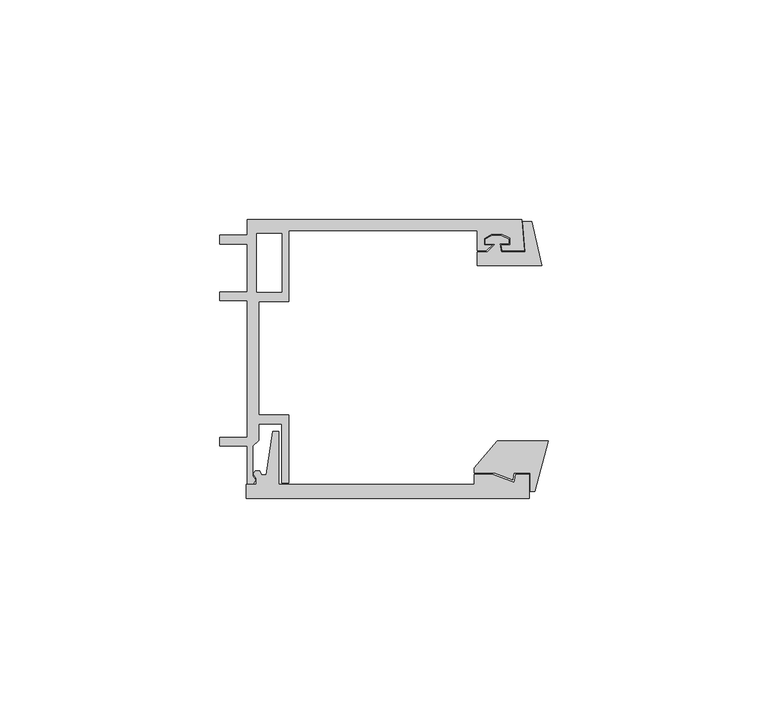
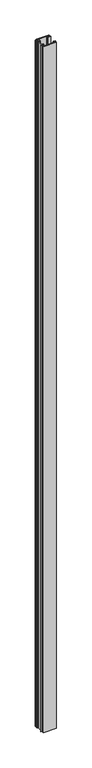
"""IFC4 building model written with IfcOpenShell, lengths in millimetres: proxy geometry, Generic Models 2:Generic Models 2:310765:Generic Models 2:310765 : Generic Models 2:Generic Models 2:310765:69 : Generic Models 2:Generic Models 2:310765:Generic Models 2:310765 : Generic Models 2:Generic Models 2:310765:300385."""

from ifc_helpers import new_model, si_unit, frame, origin, place, context, project, spatial, polyline, outline, extrude, source, transform, mapped, element, save


def generic_models_3473c4d2(model_context):
    return source(origin(), model_context, "Body", "SweptSolid", [
        extrude(outline(polyline([(596192.2839587, -579078.5739799), (596192.7605868, -579079.4334593), (596193.8113738, -579079.4334593), (596195.2258729, -579069.5319653), (596196.5980218, -579069.5319653), (596196.5980218, -579081.6864938), (596241.1250993, -579081.6864938), (596241.1250993, -579079.3741689), (596245.3940068, -579079.3741689), (596250.2558182, -579081.1528804), (596250.5522702, -579079.3741689), (596253.6946604, -579079.3741689), (596253.6946604, -579084.8288841), (596189.1867239, -579084.8288841), (596189.1867239, -579081.6864938), (596191.4990489, -579081.6864938), (596191.4990489, -579080.2786171), (596190.8403865, -579079.2652904), (596191.3340898, -579078.5247354), (596192.2839587, -579078.5739799)])), frame((0.0, 0.0, 1989.1494403), z_axis=(0.0, 0.0, 1.0), x_axis=(1.0, 0.0, 0.0)), (0.0, 0.0, 1.0), 3670.2203961),
        extrude(outline(polyline([(596254.9309933, -579083.2164454), (596253.8923802, -579083.2164454), (596253.8923802, -579079.0835833), (596250.1261424, -579079.0835833), (596249.8691362, -579080.6256201), (596245.6542355, -579079.0835833), (596241.1250993, -579079.0835833), (596241.1250993, -579077.8782793), (596246.3737657, -579071.7849999), (596257.9793788, -579071.7849999), (596254.9309933, -579083.2164454)])), frame((0.0, 0.0, 1989.1494403), z_axis=(0.0, 0.0, 1.0), x_axis=(1.0, 0.0, 0.0)), (0.0, 0.0, 1.0), 3670.2203961),
        extrude(outline(polyline([(596241.8365839, -579023.8783705), (596198.9103467, -579023.8783705), (596198.9103467, -579039.9460643), (596192.0326623, -579039.9460643), (596192.0326623, -579065.8559616), (596198.9103467, -579065.8559616), (596198.9103467, -579081.3307515), (596197.3687968, -579081.3307515), (596197.3687968, -579067.8718346), (596192.0326623, -579067.8718346), (596192.0326623, -579071.6071287), (596190.7282739, -579072.9115171), (596190.7282739, -579079.7299112), (596191.3804681, -579080.6785573), (596190.8468547, -579081.5086227), (596189.4831758, -579081.5086227), (596189.4831758, -579072.9115171), (596183.1983953, -579072.9115171), (596183.1983953, -579070.8956441), (596189.4831758, -579070.8956441), (596189.4831758, -579039.8274835), (596183.1983953, -579039.8274835), (596183.1983953, -579037.8116105), (596189.4831758, -579037.8116105), (596189.4831758, -579026.9021801), (596183.1983953, -579026.9021801), (596183.1983953, -579024.8863071), (596189.4831758, -579024.8863071), (596189.4831758, -579021.3288841), (596251.9104078, -579021.3288841), (596252.5088528, -579028.44373), (596247.4691702, -579028.44373), (596247.2464698, -579027.1393416), (596249.2796933, -579027.1393416), (596249.2796933, -579025.5486834), (596247.3809002, -579024.6632617), (596245.0994812, -579024.6632617), (596243.3781338, -579025.657082), (596243.3781338, -579027.1393416), (596245.186451, -579027.1393416), (596243.8821785, -579028.44373), (596241.8365839, -579028.44373), (596241.8365839, -579023.8783705)]), holes=[polyline([(596191.6176296, -579024.4712744), (596191.6176296, -579037.8116105), (596197.3687968, -579037.8116105), (596197.3687968, -579024.4712744), (596191.6176296, -579024.4712744)])]), frame((0.0, 0.0, 1989.1494403), z_axis=(0.0, 0.0, 1.0), x_axis=(1.0, 0.0, 0.0)), (0.0, 0.0, 1.0), 3670.2203961),
        extrude(outline(polyline([(596256.4892027, -579031.7849999), (596241.8365839, -579031.7849999), (596241.8365839, -579028.7505755), (596244.0648238, -579028.7505755), (596245.9032352, -579026.9121641), (596243.648847, -579026.9121641), (596243.648847, -579025.8229772), (596245.1391873, -579024.9625289), (596247.2194858, -579024.9625289), (596249.0209693, -579025.8025744), (596249.0209693, -579026.8269234), (596246.982706, -579026.8269234), (596247.3111344, -579028.7505755), (596252.7514342, -579028.7505755), (596252.1690236, -579021.8263604), (596254.2704385, -579021.8263604), (596256.4892027, -579031.7849999)])), frame((0.0, 0.0, 1989.1494403), z_axis=(0.0, 0.0, 1.0), x_axis=(1.0, 0.0, 0.0)), (0.0, 0.0, 1.0), 3670.2203961),
    ])


if __name__ == "__main__":
    model = new_model("IFC4")
    model_context = context("Model", 3, world=origin())
    ifc_project = project(units=[si_unit("LENGTHUNIT", "METRE", prefix="MILLI")], contexts=[model_context])
    site = spatial("IfcSite", under=ifc_project)
    building = spatial("IfcBuilding", under=site)
    placement = place(None, origin())
    generic_models_shape = generic_models_3473c4d2(model_context)
    element("IfcBuildingElementProxy", 1, Name="Generic Models 2:Generic Models 2:310765:Generic Models 2:310765 : Generic Models 2:Generic Models 2:310765:69 : Generic Models 2:Generic Models 2:310765:Generic Models 2:310765 : Generic Models 2:Generic Models 2:310765:300385", ObjectType="Generic Models 2:Generic Models 2:310765:Generic Models 2:310765 : Generic Models 2:Generic Models 2:310765:69 : Generic Models 2:Generic Models 2:310765:Generic Models 2:310765 : Generic Models 2:Generic Models 2:310765:300385", at=placement, inside=building, context=model_context, shape_type="MappedRepresentation", body=[
        mapped(generic_models_shape, transform((0.0, 0.0, 0.0), x_axis=(1.0, 0.0, 0.0), y_axis=(0.0, 1.0, 0.0), z_axis=(0.0, 0.0, 1.0))),
    ])
    save(model, "model.ifc")

# Revit data of these elements
# Type "Generic Models 2:Generic Models 2:310765:Generic Models 2:310765 : Generic Models 2:Generic Models 2:310765:69 : Generic Models 2:Generic Models 2:310765:Generic Models 2:310765 : Generic Models 2:Generic Models 2:310765:300385"
#   NameOverride = "Generic Models 2:Generic Models 2:310765:Generic Models 2:310765 : Generic Models 2:Generic Models 2:310765:300385"
#   ObjectTypeOverride = "Generic Models 2:310765 : Generic Models 2:Generic Models 2:310765"
#   Reference = "Generic Models 2"
#   Tag = "300385"
# Element 1 (IfcBuildingElementProxy, "Generic Models 2:Generic Models 2:310765:Generic Models 2:310765 : Generic Models 2:Generic Models 2:310765:69 : Generic Models 2:Generic Models 2:310765:Generic Models 2:310765 : Generic Models 2:Generic Models 2:310765:300385")
#   Materials on its faces: "THERMAL BROKEN ALUMINUM STOREFRONT FOR POLYCARBONATE"
# Materials
#   "THERMAL BROKEN ALUMINUM STOREFRONT FOR POLYCARBONATE": class "Unassigned", colour RGB 244 244 244, transparency 0, Keynote = "M07611300.01", Cost = 0
